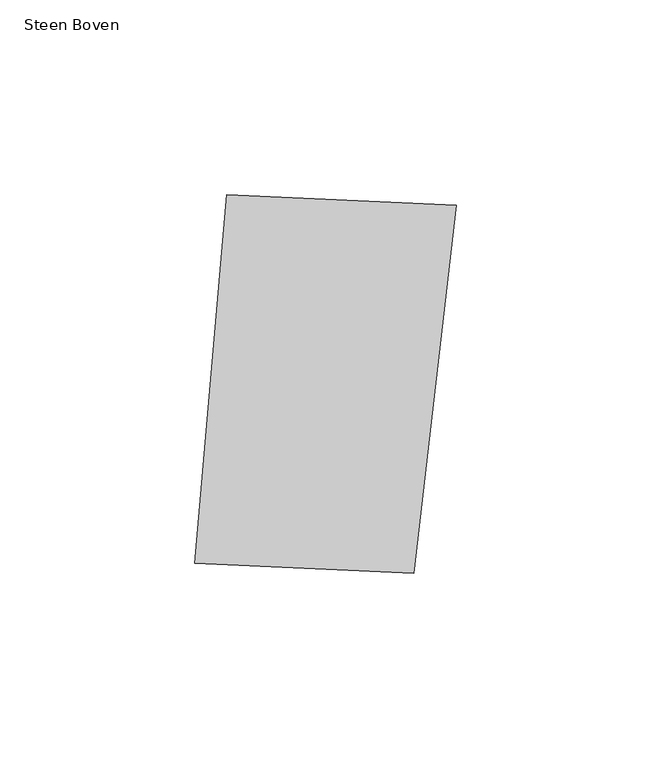
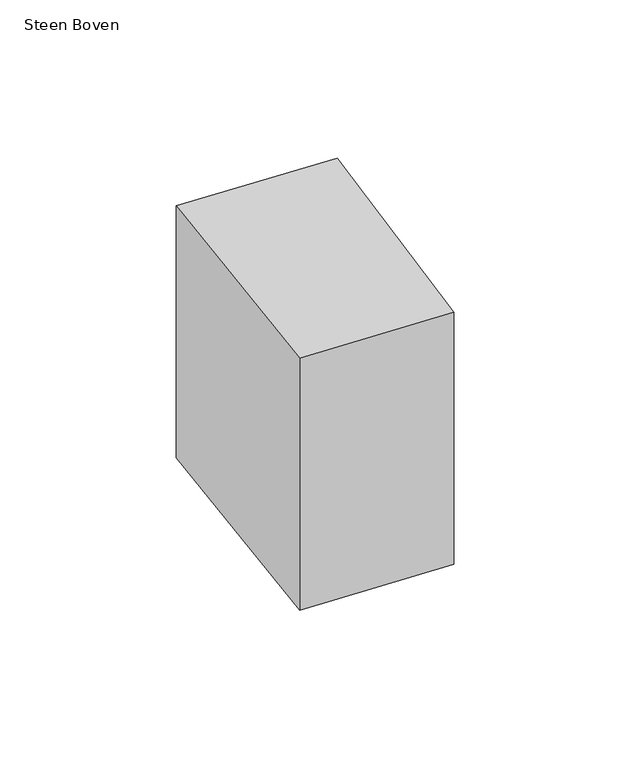
"""IFC4 building model written with IfcOpenShell, lengths in millimetres: proxy geometry, 00_GMA_steen_versie_4 : Steen Boven."""

from ifc_helpers import new_model, si_unit, origin, origin_with_axes, place, context, project, spatial, polyline, outline, extrude, source, transform, mapped, element, save


def steen_boven_26140218(model_context):
    return source(origin(), model_context, "Body", "SweptSolid", [
        extrude(outline(polyline([(106.3172402, 118.6145349), (95.374274, 24.0083503), (39.0907656, 26.6225769), (47.4149135, 121.3436608), (106.3172402, 118.6145349)])), origin_with_axes(), (0.0, 0.0, 1.0), 100.0),
    ])


if __name__ == "__main__":
    model = new_model("IFC4")
    model_context = context("Model", 3, world=origin())
    ifc_project = project(units=[si_unit("LENGTHUNIT", "METRE", prefix="MILLI")], contexts=[model_context])
    site = spatial("IfcSite", under=ifc_project)
    building = spatial("IfcBuilding", under=site)
    placement = place(None, origin())
    steen_boven_shape = steen_boven_26140218(model_context)
    element("IfcBuildingElementProxy", 1, Name="00_GMA_steen_versie_4 : Steen Boven", ObjectType="00_GMA_steen_versie_4 : Steen Boven", at=placement, inside=building, context=model_context, shape_type="MappedRepresentation", body=[
        mapped(steen_boven_shape, transform((0.0, 0.0, 0.0), x_axis=(1.0, 0.0, 0.0), y_axis=(0.0, 1.0, 0.0), z_axis=(0.0, 0.0, 1.0))),
    ])
    save(model, "model.ifc")

# Revit data of these elements
# Type "00_GMA_steen_versie_4 : Steen Boven"
#   StootVoegHalfBoven [instance default] = 5 mm
#   StootVoegHalf [instance default] = 5 mm
#   StootVoegBreedteOnder = 10 mm
#   StootVoegBreedteBoven = 10 mm
#   Steendikte = 100 mm
#   LintVoegOnderHalf = 5 mm
#   LintVoegOnder = 10 mm
#   LintVoegBovenHalf = 0 mm
#   LintVoegBoven = 0 mm
#   materiaal = none
#   MateriaalVoeg = none
#   Default Elevation = 0
